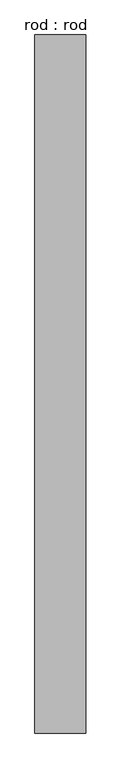
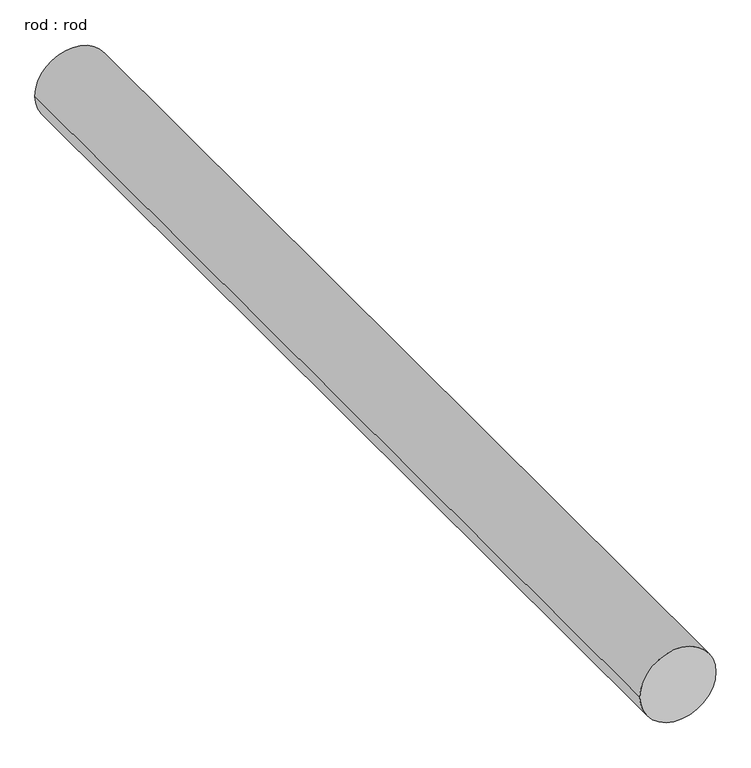
"""IFC4 building model written with IfcOpenShell, lengths in millimetres: proxy geometry, rod : rod."""

from ifc_helpers import new_model, si_unit, point, frame, frame_2d, origin, place, context, project, spatial, circle_curve, trimmed, segment, composite_curve, outline, extrude, source, transform, mapped, element, save


def rod_rod_1ae05502(model_context):
    return source(origin(), model_context, "Body", "SweptSolid", [
        extrude(outline(composite_curve([segment(trimmed(circle_curve(frame_2d((0.0108462, 0.0)), 200.0), [point((0.0108462, 200.0))], [point((0.0108462, -200.0))], False, "CARTESIAN"), True, "CONTINUOUS"), segment(trimmed(circle_curve(frame_2d((0.0108462, 0.0)), 200.0), [point((0.0108462, -200.0))], [point((0.0108462, 200.0))], False, "CARTESIAN"), True, "CONTINUOUS")], self_intersect=False)), frame((0.0, 1339.9317422, 0.0), z_axis=(0.0, 1.0, 0.0), x_axis=(0.0, 0.0, 1.0)), (0.0, 0.0, 1.0), 5505.5937464),
    ])


if __name__ == "__main__":
    model = new_model("IFC4")
    model_context = context("Model", 3, world=origin())
    ifc_project = project(units=[si_unit("LENGTHUNIT", "METRE", prefix="MILLI")], contexts=[model_context])
    site = spatial("IfcSite", under=ifc_project)
    building = spatial("IfcBuilding", under=site)
    placement = place(None, origin())
    rod_rod_shape = rod_rod_1ae05502(model_context)
    element("IfcBuildingElementProxy", 1, Name="rod : rod", ObjectType="rod : rod", at=placement, inside=building, context=model_context, shape_type="MappedRepresentation", body=[
        mapped(rod_rod_shape, transform((0.0, 0.0, 0.0), x_axis=(1.0, 0.0, 0.0), y_axis=(0.0, 1.0, 0.0), z_axis=(0.0, 0.0, 1.0))),
    ])
    save(model, "model.ifc")

# Revit data of these elements
# Type "rod : rod"
#   Default Elevation = 0
